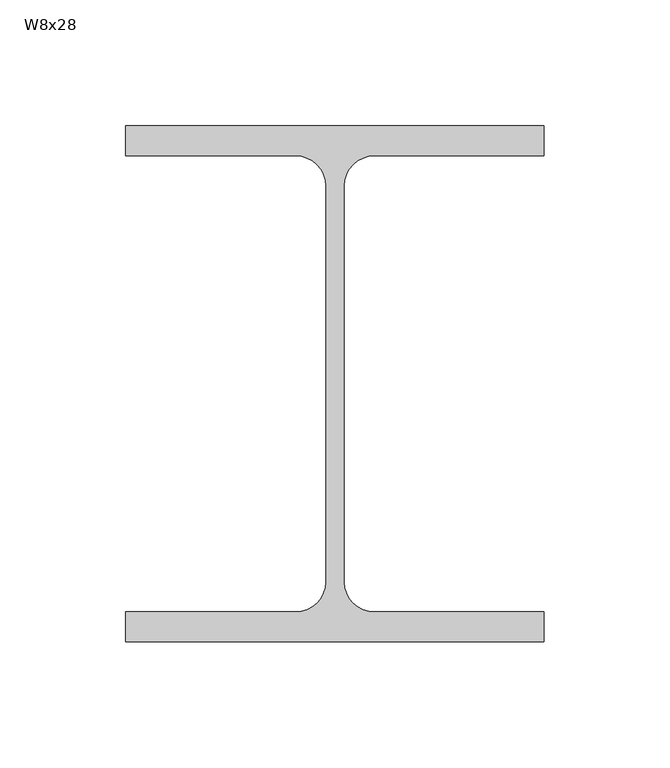
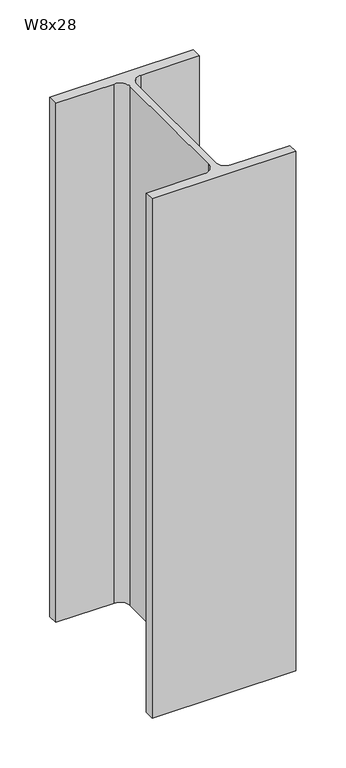
"""IFC4 building model written with IfcOpenShell, lengths in millimetres: column geometry, RME WF - Column : W8x28."""

from ifc_helpers import new_model, si_unit, point, frame, frame_2d, origin, place, context, project, spatial, polyline, circle_curve, trimmed, segment, composite_curve, outline, extrude, source, transform, mapped, element, save


def w8x28_840d24c1(model_context):
    return source(origin(), model_context, "Body", "SweptSolid", [
        extrude(outline(composite_curve([segment(polyline([(83.058, 102.362), (83.058, 90.551), (15.621, 90.551)]), True, "CONTINUOUS"), segment(trimmed(circle_curve(frame_2d((15.621, 78.5495)), 12.0015), [point((15.621, 90.551))], [point((3.6195, 78.5495))], True, "CARTESIAN"), True, "CONTINUOUS"), segment(polyline([(3.6195, 78.5495), (3.6195, -78.5495)]), True, "CONTINUOUS"), segment(trimmed(circle_curve(frame_2d((15.621, -78.5495)), 12.0015), [point((3.6195, -78.5495))], [point((15.621, -90.551))], True, "CARTESIAN"), True, "CONTINUOUS"), segment(polyline([(15.621, -90.551), (83.058, -90.551), (83.058, -102.362), (-83.058, -102.362), (-83.058, -90.551), (-15.621, -90.551)]), True, "CONTINUOUS"), segment(trimmed(circle_curve(frame_2d((-15.621, -78.5495)), 12.0015), [point((-15.621, -90.551))], [point((-3.6195, -78.5495))], True, "CARTESIAN"), True, "CONTINUOUS"), segment(polyline([(-3.6195, -78.5495), (-3.6195, 78.5495)]), True, "CONTINUOUS"), segment(trimmed(circle_curve(frame_2d((-15.621, 78.5495)), 12.0015), [point((-3.6195, 78.5495))], [point((-15.621, 90.551))], True, "CARTESIAN"), True, "CONTINUOUS"), segment(polyline([(-15.621, 90.551), (-83.058, 90.551), (-83.058, 102.362), (83.058, 102.362)]), True, "CONTINUOUS")], self_intersect=False)), frame((0.0, 0.0, 4679.95), z_axis=(0.0, 0.0, 1.0), x_axis=(1.0, 0.0, 0.0)), (0.0, 0.0, 1.0), 635.0),
    ])


if __name__ == "__main__":
    model = new_model("IFC4")
    model_context = context("Model", 3, world=origin())
    ifc_project = project(units=[si_unit("LENGTHUNIT", "METRE", prefix="MILLI")], contexts=[model_context])
    site = spatial("IfcSite", under=ifc_project)
    building = spatial("IfcBuilding", under=site)
    placement = place(None, origin())
    w8x28_shape = w8x28_840d24c1(model_context)
    element("IfcColumn", 1, ObjectType="RME WF - Column : W8x28", at=placement, inside=building, context=model_context, shape_type="MappedRepresentation", body=[
        mapped(w8x28_shape, transform((0.0, 0.0, 0.0), x_axis=(1.0, 0.0, 0.0), y_axis=(0.0, 1.0, 0.0), z_axis=(0.0, 0.0, 1.0))),
    ])
    save(model, "model.ifc")

# Revit data of these elements
# Type "RME WF - Column : W8x28"
#   REINF TYPE [instance default] = ""
#   Nominal Size = "W16"
#   COL REMARKS [instance default] = ""
#   BP [instance default] = ""
#   Assembly Code = "B10"
#   W = 28
#   bf = 0' - 6.54"
#   d = 0' - 8.06"
#   k = 0' - 0 15/16"
#   kr = 0' - 0.4725"
#   tf = 0' - 0.465"
#   tw = 0' - 0.285"
#   A = 0.0572222 SF
#   Structural Material [instance default] = Metal - Steel - ASTM A992
# Element 1 (IfcColumn, "RME WF - Column : W8x28")
#   Materials on its faces: "Metal - Steel - ASTM A992"
# Materials
#   "Metal - Steel - ASTM A992": class "Metal", colour RGB 255 128 0, transparency 0
